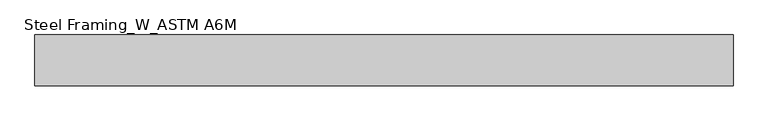
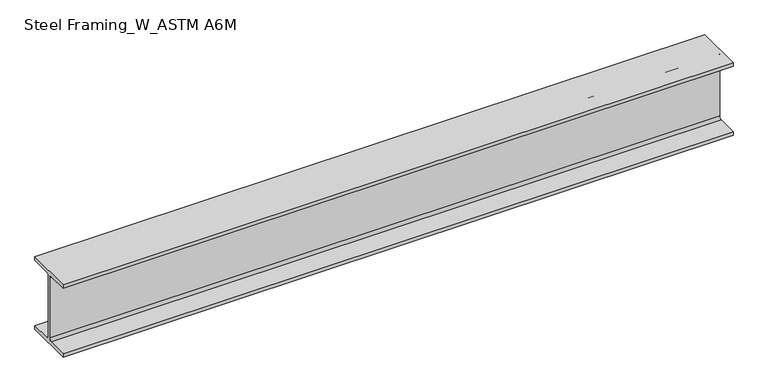
"""IFC4 building model written with IfcOpenShell, lengths in millimetres: beam geometry, Steel Framing_W_ASTM A6M : H_SB_AR_S02_W200x31.3_B6."""

import ifcopenshell
import ifcopenshell.guid

model = None  # the IFC model being written
_history = None  # IfcOwnerHistory: only IFC2X3 demands one
_inside = {}  # id of a spatial element -> (the spatial element, [elements in it])
_under = {}  # id of a project, library or spatial element -> (it, [spatial elements below it])
_declared = {}  # id of a project -> (the project, [libraries it declares])
_typed = {}  # id of a type object -> (the type object, [elements of that type])
_made_of = {}  # id of a material, layer set ... -> (it, [elements and type objects made of it])


def new_model(schema):
    """Start an empty IFC model of exactly this schema.

    Asked for "IFC4X3", IfcOpenShell would pick the latest addendum, in which some entities
    have other attributes; the version numbers below select the first issue.
    IFC2X3 requires an IfcOwnerHistory on every rooted entity: one is made here for all.
    """
    global model, _history
    if schema == "IFC4X3":
        model = ifcopenshell.file(schema_version=(4, 3, 0, 0))
    else:
        model = ifcopenshell.file(schema=schema)
    _inside.clear()
    _under.clear()
    _declared.clear()
    _typed.clear()
    _made_of.clear()
    _history = None
    if model.schema == "IFC2X3":
        org = make("IfcOrganization", Name="unknown")
        user = make(
            "IfcPersonAndOrganization",
            ThePerson=make("IfcPerson", FamilyName="unknown"),
            TheOrganization=org,
        )
        app = make(
            "IfcApplication",
            ApplicationDeveloper=org,
            Version="unknown",
            ApplicationFullName="unknown",
            ApplicationIdentifier="unknown",
        )
        _history = make(
            "IfcOwnerHistory",
            OwningUser=user,
            OwningApplication=app,
            ChangeAction="ADDED",
            CreationDate=0,
        )
    return model


def make(cls, **values):
    """One entity of the class cls with the attributes given. An attribute that is None is left unset."""
    return model.create_entity(
        cls, **{name: value for name, value in values.items() if value is not None}
    )


def rooted(cls, **values):
    """An entity with a GlobalId (a new one), such as an element, a storey or a relation."""
    return make(cls, GlobalId=ifcopenshell.guid.new(), OwnerHistory=_history, **values)


def si_unit(unit_type, name, prefix=None):
    """IfcSIUnit, for example si_unit("LENGTHUNIT", "METRE", prefix="MILLI")."""
    return make("IfcSIUnit", UnitType=unit_type, Prefix=prefix, Name=name)


def assignment(units):
    """IfcUnitAssignment: the units of a project."""
    return None if units is None else make("IfcUnitAssignment", Units=units)


def point(xyz):
    """IfcCartesianPoint."""
    return None if xyz is None else make("IfcCartesianPoint", Coordinates=xyz)


def direction(xyz):
    """IfcDirection."""
    return None if xyz is None else make("IfcDirection", DirectionRatios=xyz)


def frame(location, z_axis=None, x_axis=None):
    """IfcAxis2Placement3D, a coordinate frame: its origin and axes. An axis left out is left unset."""
    return make(
        "IfcAxis2Placement3D",
        Location=point(location),
        Axis=direction(z_axis),
        RefDirection=direction(x_axis),
    )


def frame_2d(location, x_axis=None):
    """IfcAxis2Placement2D, a coordinate frame in the plane: its origin and x axis."""
    return make(
        "IfcAxis2Placement2D", Location=point(location), RefDirection=direction(x_axis)
    )


def origin():
    """The frame at (0, 0, 0) with its axes left unset."""
    return frame((0.0, 0.0, 0.0))


def place(relative_to, where):
    """IfcLocalPlacement: puts the frame where relative to a parent placement (None: the world)."""
    return make(
        "IfcLocalPlacement", PlacementRelTo=relative_to, RelativePlacement=where
    )


def context(
    kind, dimensions, precision=None, world=None, true_north=None, identifier=None
):
    """IfcGeometricRepresentationContext, for example the 3D "Model" context."""
    return make(
        "IfcGeometricRepresentationContext",
        ContextIdentifier=identifier,
        ContextType=kind,
        CoordinateSpaceDimension=dimensions,
        Precision=precision,
        WorldCoordinateSystem=world,
        TrueNorth=true_north,
    )


def project(units=None, contexts=None):
    """IfcProject with its units and contexts."""
    return rooted(
        "IfcProject",
        Name="project",
        RepresentationContexts=contexts,
        UnitsInContext=assignment(units),
    )


def spatial(cls, under=None, at=None, **own):
    """A site, building, storey or space (cls), placed at a placement, below another one or the project."""
    s = rooted(cls, ObjectPlacement=at, **own)
    if under is not None:
        _under.setdefault(under.id(), (under, []))[1].append(s)
    return s


def polyline(points):
    """IfcPolyline through the points."""
    return make("IfcPolyline", Points=[point(p) for p in points])


def circle_curve(where, radius):
    """IfcCircle in the frame where."""
    return make("IfcCircle", Position=where, Radius=radius)


def trimmed(basis, trim1, trim2, sense, master):
    """IfcTrimmedCurve: the piece of a basis curve between two trims."""
    return make(
        "IfcTrimmedCurve",
        BasisCurve=basis,
        Trim1=trim1,
        Trim2=trim2,
        SenseAgreement=sense,
        MasterRepresentation=master,
    )


def segment(curve, same_sense, transition):
    """IfcCompositeCurveSegment."""
    return make(
        "IfcCompositeCurveSegment",
        Transition=transition,
        SameSense=same_sense,
        ParentCurve=curve,
    )


def composite_curve(segments, self_intersect=None):
    """IfcCompositeCurve: segments joined end to end."""
    return make("IfcCompositeCurve", Segments=segments, SelfIntersect=self_intersect)


def outline(outer, holes=None, kind="AREA"):
    """IfcArbitraryClosedProfileDef: a profile drawn as a closed curve; with holes, ...WithVoids."""
    if holes is None:
        return make("IfcArbitraryClosedProfileDef", ProfileType=kind, OuterCurve=outer)
    return make(
        "IfcArbitraryProfileDefWithVoids",
        ProfileType=kind,
        OuterCurve=outer,
        InnerCurves=holes,
    )


def extrude(swept, where, along, depth):
    """IfcExtrudedAreaSolid: the profile swept, set in the frame where, extruded along a direction by depth."""
    return make(
        "IfcExtrudedAreaSolid",
        SweptArea=swept,
        Position=where,
        ExtrudedDirection=direction(along),
        Depth=depth,
    )


def shape(context_of_items, identifier, shape_type, items):
    """IfcShapeRepresentation: the items that make up one representation, for example the "Body"."""
    return make(
        "IfcShapeRepresentation",
        ContextOfItems=context_of_items,
        RepresentationIdentifier=identifier,
        RepresentationType=shape_type,
        Items=items,
    )


def source(mapping_origin, context_of_items, identifier, shape_type, items):
    """IfcRepresentationMap: a shape defined once, which mapped items show again and again."""
    return make(
        "IfcRepresentationMap",
        MappingOrigin=mapping_origin,
        MappedRepresentation=shape(context_of_items, identifier, shape_type, items),
    )


def transform(
    local_origin,
    x_axis=None,
    y_axis=None,
    z_axis=None,
    scale=None,
    scale2=None,
    scale3=None,
    uniform=True,
):
    """IfcCartesianTransformationOperator3D, or its non-uniform kind. x_axis, y_axis, z_axis: its Axis1, 2, 3."""
    if uniform:
        return make(
            "IfcCartesianTransformationOperator3D",
            Axis1=direction(x_axis),
            Axis2=direction(y_axis),
            LocalOrigin=point(local_origin),
            Scale=scale,
            Axis3=direction(z_axis),
        )
    return make(
        "IfcCartesianTransformationOperator3DnonUniform",
        Axis1=direction(x_axis),
        Axis2=direction(y_axis),
        LocalOrigin=point(local_origin),
        Scale=scale,
        Axis3=direction(z_axis),
        Scale2=scale2,
        Scale3=scale3,
    )


def mapped(mapping_source, mapping_target):
    """IfcMappedItem: shows the shape of a source again, moved by a transform."""
    return make(
        "IfcMappedItem", MappingSource=mapping_source, MappingTarget=mapping_target
    )


def made_of(thing, what):
    """Note that an element or type object is made of a material, layer set ...; save() writes the relation."""
    if what is not None:
        _made_of.setdefault(what.id(), (what, []))[1].append(thing)
    return thing


def element(
    cls,
    number,
    at=None,
    inside=None,
    cuts=None,
    type_object=None,
    material=None,
    context=None,
    identifier="Body",
    shape_type=None,
    held_by="IfcProductDefinitionShape",
    body=None,
    shapes=None,
    **own,
):
    """One element of the class cls, such as IfcWall. Its Tag is "e" and its number.

    at: its placement. inside: the storey or other place that contains it. cuts: it is an
    opening in that element (IfcRelVoidsElement). A single representation is given by context,
    identifier, shape_type and body (its items); several are given by shapes. held_by: the class
    of the entity that holds the representations. save() writes the other relations.
    """
    e = rooted(cls, Tag="e%d" % number, ObjectPlacement=at, **own)
    if body is not None:
        shapes = [shape(context, identifier, shape_type, body)]
    if shapes is not None:
        e.Representation = make(held_by, Representations=shapes)
    if inside is not None:
        _inside.setdefault(inside.id(), (inside, []))[1].append(e)
    if cuts is not None:
        rooted(
            "IfcRelVoidsElement", RelatingBuildingElement=cuts, RelatedOpeningElement=e
        )
    if type_object is not None:
        _typed.setdefault(type_object.id(), (type_object, []))[1].append(e)
    return made_of(e, material)


def aggregate(whole, parts):
    """IfcRelAggregates: a whole, such as a stair, and the parts it consists of."""
    return rooted("IfcRelAggregates", RelatingObject=whole, RelatedObjects=parts)


def save(model, path):
    """Write the relations noted so far, then the file.

    IfcRelAggregates (storeys below a building ...), IfcRelContainedInSpatialStructure (elements
    in a storey), IfcRelDefinesByType, IfcRelAssociatesMaterial and IfcRelDeclares: one each for
    every whole, place, type object, material and project.
    """
    for whole, parts in _under.values():
        aggregate(whole, parts)
    for where, things in _inside.values():
        rooted(
            "IfcRelContainedInSpatialStructure",
            RelatedElements=things,
            RelatingStructure=where,
        )
    for kind, things in _typed.values():
        rooted("IfcRelDefinesByType", RelatedObjects=things, RelatingType=kind)
    for what, things in _made_of.values():
        rooted("IfcRelAssociatesMaterial", RelatedObjects=things, RelatingMaterial=what)
    for by, libraries in _declared.values():
        rooted("IfcRelDeclares", RelatingContext=by, RelatedDefinitions=libraries)
    model.write(path)


def steel_framing_w_astm_a6m_7ac08ae9(model_context):
    return source(origin(), model_context, "Body", "SweptSolid", [
        extrude(outline(composite_curve([segment(polyline([(67.0, -94.8), (67.0, -105.0), (-67.0, -105.0), (-67.0, -94.8), (-10.775, -94.8)]), True, "CONTINUOUS"), segment(trimmed(circle_curve(frame_2d((-10.775, -87.2)), 7.6), [point((-10.775, -94.8))], [point((-3.175, -87.2))], True, "CARTESIAN"), True, "CONTINUOUS"), segment(polyline([(-3.175, -87.2), (-3.175, 87.2)]), True, "CONTINUOUS"), segment(trimmed(circle_curve(frame_2d((-10.775, 87.2)), 7.6), [point((-3.175, 87.2))], [point((-10.775, 94.8))], True, "CARTESIAN"), True, "CONTINUOUS"), segment(polyline([(-10.775, 94.8), (-67.0, 94.8), (-67.0, 105.0), (67.0, 105.0), (67.0, 94.8), (10.775, 94.8)]), True, "CONTINUOUS"), segment(trimmed(circle_curve(frame_2d((10.775, 87.2)), 7.6), [point((10.775, 94.8))], [point((3.175, 87.2))], True, "CARTESIAN"), True, "CONTINUOUS"), segment(polyline([(3.175, 87.2), (3.175, -87.2)]), True, "CONTINUOUS"), segment(trimmed(circle_curve(frame_2d((10.775, -87.2)), 7.6), [point((3.175, -87.2))], [point((10.775, -94.8))], True, "CARTESIAN"), True, "CONTINUOUS"), segment(polyline([(10.775, -94.8), (67.0, -94.8)]), True, "CONTINUOUS")], self_intersect=False)), frame((-920.3, 0.0, 0.0), z_axis=(1.0, 0.0, 0.0), x_axis=(0.0, 1.0, 0.0)), (0.0, 0.0, 1.0), 1840.6),
    ])


if __name__ == "__main__":
    model = new_model("IFC4")
    model_context = context("Model", 3, world=origin())
    ifc_project = project(units=[si_unit("LENGTHUNIT", "METRE", prefix="MILLI")], contexts=[model_context])
    site = spatial("IfcSite", under=ifc_project)
    building = spatial("IfcBuilding", under=site)
    placement = place(None, origin())
    steel_framing_w_astm_a6m_shape = steel_framing_w_astm_a6m_7ac08ae9(model_context)
    element("IfcBeam", 1, ObjectType="Steel Framing_W_ASTM A6M : H_SB_AR_S02_W200x31.3_B6", at=placement, inside=building, context=model_context, shape_type="MappedRepresentation", body=[
        mapped(steel_framing_w_astm_a6m_shape, transform((0.0, 0.0, 0.0), x_axis=(1.0, 0.0, 0.0), y_axis=(0.0, 1.0, 0.0), z_axis=(0.0, 0.0, 1.0))),
    ])
    save(model, "model.ifc")

# Revit data of these elements
# Type "Steel Framing_W_ASTM A6M : H_SB_AR_S02_W200x31.3_B6"
#   Type Mark = "B6"
#   Section Name Key = "W8x21"
#   Width = 13.4 cm
#   Web Thickness = 0.635 cm
#   Web Fillet = 0.76 cm
#   Warping Constant = 40800.0 cm⁶
#   Torsional Moment of Inertia = 11.70 cm⁴
#   Section Area = 39.7 cm²
#   Plastic Modulus weak axis = 93.2 cm³
#   Plastic Modulus strong axis = 334.0 cm³
#   Perimeter = 0.93 m²/m
#   Nominal Weight = 31.30 kgf/m
#   Moment of Inertia weak axis = 407.00 cm⁴
#   Moment of Inertia strong axis = 3130.00 cm⁴
#   Height = 21.0 cm
#   Flange Thickness = 1.02 cm
#   Elastic Modulus weak axis = 60.8 cm³
#   Elastic Modulus strong axis = 298.0 cm³
#   Centroid Vertical = 10.5 cm
#   Centroid Horizontal = 6.7 cm
#   Length [instance default] = 1500 mm
#   Structural Material [instance default] = Steel, 45-345
#   Bolt Spacing = 0
#   Assembly Code = ""
# Element 1 (IfcBeam, "Steel Framing_W_ASTM A6M : H_SB_AR_S02_W200x31.3_B6")
#   Materials on its faces: "Steel, 45-345"
# Materials
#   "Steel, 45-345": class "Metal", colour RGB 189 187 185, transparency 0, Description = "Steel 345 MPa", Cost = 0
